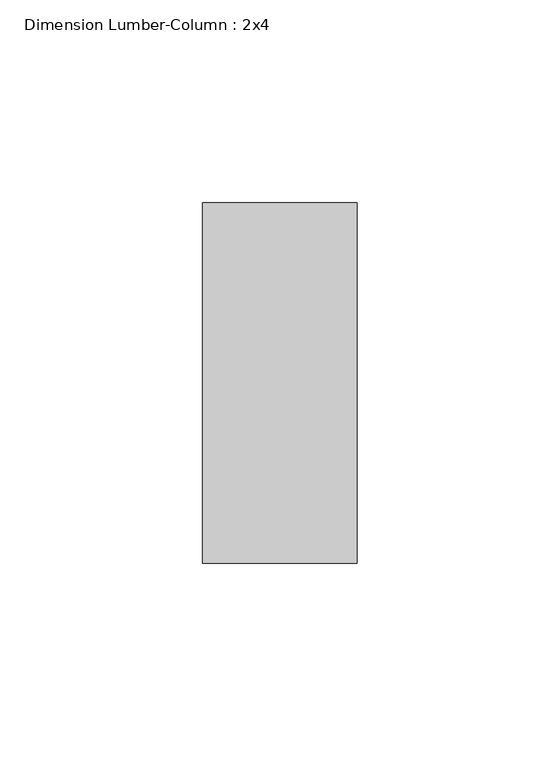
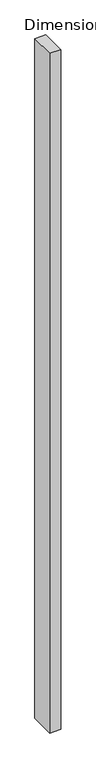
"""IFC4 building model written with IfcOpenShell, lengths in millimetres: column geometry, Dimension Lumber-Column : 2x4."""

from ifc_helpers import new_model, si_unit, frame, origin, place, context, project, spatial, polyline, outline, extrude, source, transform, mapped, element, save


def dimension_lumber_column_2x4_a0a2a51b(model_context):
    return source(origin(), model_context, "Body", "SweptSolid", [
        extrude(outline(polyline([(19.05, -44.45), (-19.05, -44.45), (-19.05, 44.45), (19.05, 44.45), (19.05, -44.45)])), frame((0.0, 0.0, 56.35625), z_axis=(0.0, 0.0, 1.0), x_axis=(1.0, 0.0, 0.0)), (0.0, 0.0, 1.0), 2477.29375),
    ])


if __name__ == "__main__":
    model = new_model("IFC4")
    model_context = context("Model", 3, world=origin())
    ifc_project = project(units=[si_unit("LENGTHUNIT", "METRE", prefix="MILLI")], contexts=[model_context])
    site = spatial("IfcSite", under=ifc_project)
    building = spatial("IfcBuilding", under=site)
    placement = place(None, origin())
    dimension_lumber_column_2x4_shape = dimension_lumber_column_2x4_a0a2a51b(model_context)
    element("IfcColumn", 1, ObjectType="Dimension Lumber-Column : 2x4", at=placement, inside=building, context=model_context, shape_type="MappedRepresentation", body=[
        mapped(dimension_lumber_column_2x4_shape, transform((0.0, 0.0, 0.0), x_axis=(1.0, 0.0, 0.0), y_axis=(0.0, 1.0, 0.0), z_axis=(0.0, 0.0, 1.0))),
    ])
    save(model, "model.ifc")

# Revit data of these elements
# Type "Dimension Lumber-Column : 2x4"
#   Int Type = "Interior"
#   Assembly Code = "B10"
#   Cost = 8.05
#   A = 0.0364583 SF
#   b = 0' - 1 1/2"
#   d = 0' - 3 1/2"
#   Structural Material [instance default] = Softwood, Lumber
# Element 1 (IfcColumn, "Dimension Lumber-Column : 2x4")
#   Structural Material = Douglas Fir #2
#   Materials on its faces: "Douglas Fir #2"
# Materials
#   "Softwood, Lumber": class "Wood", colour RGB 223 192 134, transparency 0, Description = "Pinus Echinata", Cost = 0
#   "Douglas Fir #2": class "Wood", colour RGB 223 192 134, transparency 0, Description = "Pinus Echinata", Cost = 0
